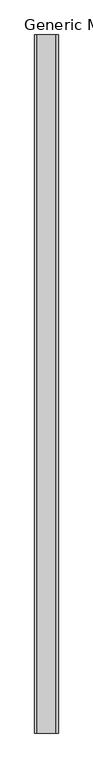
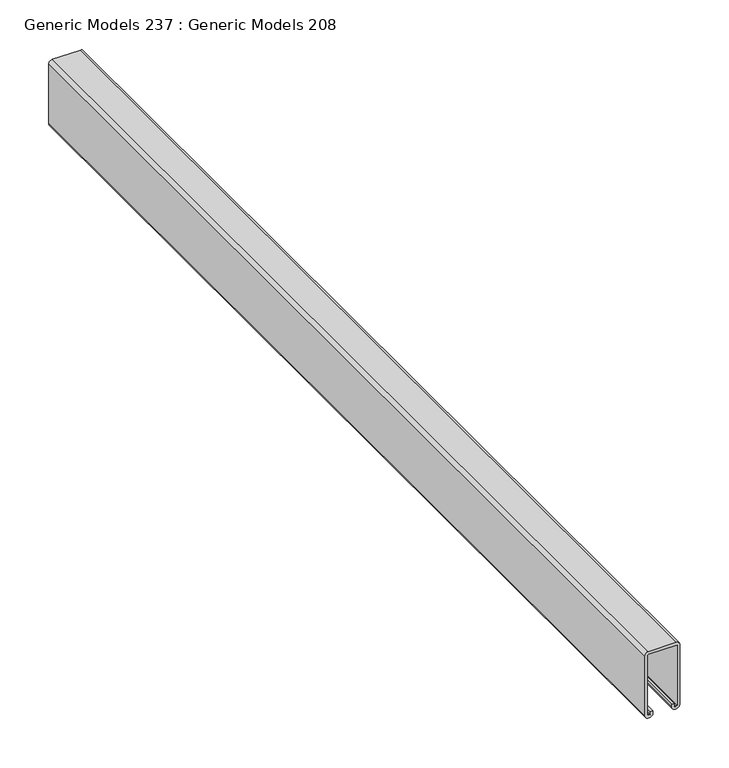
"""IFC4 building model written with IfcOpenShell, lengths in millimetres: proxy geometry, Generic Models 237 : Generic Models 208."""

import ifcopenshell
import ifcopenshell.guid

model = None  # the IFC model being written
_history = None  # IfcOwnerHistory: only IFC2X3 demands one
_inside = {}  # id of a spatial element -> (the spatial element, [elements in it])
_under = {}  # id of a project, library or spatial element -> (it, [spatial elements below it])
_declared = {}  # id of a project -> (the project, [libraries it declares])
_typed = {}  # id of a type object -> (the type object, [elements of that type])
_made_of = {}  # id of a material, layer set ... -> (it, [elements and type objects made of it])


def new_model(schema):
    """Start an empty IFC model of exactly this schema.

    Asked for "IFC4X3", IfcOpenShell would pick the latest addendum, in which some entities
    have other attributes; the version numbers below select the first issue.
    IFC2X3 requires an IfcOwnerHistory on every rooted entity: one is made here for all.
    """
    global model, _history
    if schema == "IFC4X3":
        model = ifcopenshell.file(schema_version=(4, 3, 0, 0))
    else:
        model = ifcopenshell.file(schema=schema)
    _inside.clear()
    _under.clear()
    _declared.clear()
    _typed.clear()
    _made_of.clear()
    _history = None
    if model.schema == "IFC2X3":
        org = make("IfcOrganization", Name="unknown")
        user = make(
            "IfcPersonAndOrganization",
            ThePerson=make("IfcPerson", FamilyName="unknown"),
            TheOrganization=org,
        )
        app = make(
            "IfcApplication",
            ApplicationDeveloper=org,
            Version="unknown",
            ApplicationFullName="unknown",
            ApplicationIdentifier="unknown",
        )
        _history = make(
            "IfcOwnerHistory",
            OwningUser=user,
            OwningApplication=app,
            ChangeAction="ADDED",
            CreationDate=0,
        )
    return model


def make(cls, **values):
    """One entity of the class cls with the attributes given. An attribute that is None is left unset."""
    return model.create_entity(
        cls, **{name: value for name, value in values.items() if value is not None}
    )


def rooted(cls, **values):
    """An entity with a GlobalId (a new one), such as an element, a storey or a relation."""
    return make(cls, GlobalId=ifcopenshell.guid.new(), OwnerHistory=_history, **values)


def si_unit(unit_type, name, prefix=None):
    """IfcSIUnit, for example si_unit("LENGTHUNIT", "METRE", prefix="MILLI")."""
    return make("IfcSIUnit", UnitType=unit_type, Prefix=prefix, Name=name)


def assignment(units):
    """IfcUnitAssignment: the units of a project."""
    return None if units is None else make("IfcUnitAssignment", Units=units)


def point(xyz):
    """IfcCartesianPoint."""
    return None if xyz is None else make("IfcCartesianPoint", Coordinates=xyz)


def direction(xyz):
    """IfcDirection."""
    return None if xyz is None else make("IfcDirection", DirectionRatios=xyz)


def frame(location, z_axis=None, x_axis=None):
    """IfcAxis2Placement3D, a coordinate frame: its origin and axes. An axis left out is left unset."""
    return make(
        "IfcAxis2Placement3D",
        Location=point(location),
        Axis=direction(z_axis),
        RefDirection=direction(x_axis),
    )


def frame_2d(location, x_axis=None):
    """IfcAxis2Placement2D, a coordinate frame in the plane: its origin and x axis."""
    return make(
        "IfcAxis2Placement2D", Location=point(location), RefDirection=direction(x_axis)
    )


def origin():
    """The frame at (0, 0, 0) with its axes left unset."""
    return frame((0.0, 0.0, 0.0))


def place(relative_to, where):
    """IfcLocalPlacement: puts the frame where relative to a parent placement (None: the world)."""
    return make(
        "IfcLocalPlacement", PlacementRelTo=relative_to, RelativePlacement=where
    )


def context(
    kind, dimensions, precision=None, world=None, true_north=None, identifier=None
):
    """IfcGeometricRepresentationContext, for example the 3D "Model" context."""
    return make(
        "IfcGeometricRepresentationContext",
        ContextIdentifier=identifier,
        ContextType=kind,
        CoordinateSpaceDimension=dimensions,
        Precision=precision,
        WorldCoordinateSystem=world,
        TrueNorth=true_north,
    )


def project(units=None, contexts=None):
    """IfcProject with its units and contexts."""
    return rooted(
        "IfcProject",
        Name="project",
        RepresentationContexts=contexts,
        UnitsInContext=assignment(units),
    )


def spatial(cls, under=None, at=None, **own):
    """A site, building, storey or space (cls), placed at a placement, below another one or the project."""
    s = rooted(cls, ObjectPlacement=at, **own)
    if under is not None:
        _under.setdefault(under.id(), (under, []))[1].append(s)
    return s


def polyline(points):
    """IfcPolyline through the points."""
    return make("IfcPolyline", Points=[point(p) for p in points])


def circle_curve(where, radius):
    """IfcCircle in the frame where."""
    return make("IfcCircle", Position=where, Radius=radius)


def trimmed(basis, trim1, trim2, sense, master):
    """IfcTrimmedCurve: the piece of a basis curve between two trims."""
    return make(
        "IfcTrimmedCurve",
        BasisCurve=basis,
        Trim1=trim1,
        Trim2=trim2,
        SenseAgreement=sense,
        MasterRepresentation=master,
    )


def segment(curve, same_sense, transition):
    """IfcCompositeCurveSegment."""
    return make(
        "IfcCompositeCurveSegment",
        Transition=transition,
        SameSense=same_sense,
        ParentCurve=curve,
    )


def composite_curve(segments, self_intersect=None):
    """IfcCompositeCurve: segments joined end to end."""
    return make("IfcCompositeCurve", Segments=segments, SelfIntersect=self_intersect)


def outline(outer, holes=None, kind="AREA"):
    """IfcArbitraryClosedProfileDef: a profile drawn as a closed curve; with holes, ...WithVoids."""
    if holes is None:
        return make("IfcArbitraryClosedProfileDef", ProfileType=kind, OuterCurve=outer)
    return make(
        "IfcArbitraryProfileDefWithVoids",
        ProfileType=kind,
        OuterCurve=outer,
        InnerCurves=holes,
    )


def extrude(swept, where, along, depth):
    """IfcExtrudedAreaSolid: the profile swept, set in the frame where, extruded along a direction by depth."""
    return make(
        "IfcExtrudedAreaSolid",
        SweptArea=swept,
        Position=where,
        ExtrudedDirection=direction(along),
        Depth=depth,
    )


def shape(context_of_items, identifier, shape_type, items):
    """IfcShapeRepresentation: the items that make up one representation, for example the "Body"."""
    return make(
        "IfcShapeRepresentation",
        ContextOfItems=context_of_items,
        RepresentationIdentifier=identifier,
        RepresentationType=shape_type,
        Items=items,
    )


def source(mapping_origin, context_of_items, identifier, shape_type, items):
    """IfcRepresentationMap: a shape defined once, which mapped items show again and again."""
    return make(
        "IfcRepresentationMap",
        MappingOrigin=mapping_origin,
        MappedRepresentation=shape(context_of_items, identifier, shape_type, items),
    )


def transform(
    local_origin,
    x_axis=None,
    y_axis=None,
    z_axis=None,
    scale=None,
    scale2=None,
    scale3=None,
    uniform=True,
):
    """IfcCartesianTransformationOperator3D, or its non-uniform kind. x_axis, y_axis, z_axis: its Axis1, 2, 3."""
    if uniform:
        return make(
            "IfcCartesianTransformationOperator3D",
            Axis1=direction(x_axis),
            Axis2=direction(y_axis),
            LocalOrigin=point(local_origin),
            Scale=scale,
            Axis3=direction(z_axis),
        )
    return make(
        "IfcCartesianTransformationOperator3DnonUniform",
        Axis1=direction(x_axis),
        Axis2=direction(y_axis),
        LocalOrigin=point(local_origin),
        Scale=scale,
        Axis3=direction(z_axis),
        Scale2=scale2,
        Scale3=scale3,
    )


def mapped(mapping_source, mapping_target):
    """IfcMappedItem: shows the shape of a source again, moved by a transform."""
    return make(
        "IfcMappedItem", MappingSource=mapping_source, MappingTarget=mapping_target
    )


def made_of(thing, what):
    """Note that an element or type object is made of a material, layer set ...; save() writes the relation."""
    if what is not None:
        _made_of.setdefault(what.id(), (what, []))[1].append(thing)
    return thing


def element(
    cls,
    number,
    at=None,
    inside=None,
    cuts=None,
    type_object=None,
    material=None,
    context=None,
    identifier="Body",
    shape_type=None,
    held_by="IfcProductDefinitionShape",
    body=None,
    shapes=None,
    **own,
):
    """One element of the class cls, such as IfcWall. Its Tag is "e" and its number.

    at: its placement. inside: the storey or other place that contains it. cuts: it is an
    opening in that element (IfcRelVoidsElement). A single representation is given by context,
    identifier, shape_type and body (its items); several are given by shapes. held_by: the class
    of the entity that holds the representations. save() writes the other relations.
    """
    e = rooted(cls, Tag="e%d" % number, ObjectPlacement=at, **own)
    if body is not None:
        shapes = [shape(context, identifier, shape_type, body)]
    if shapes is not None:
        e.Representation = make(held_by, Representations=shapes)
    if inside is not None:
        _inside.setdefault(inside.id(), (inside, []))[1].append(e)
    if cuts is not None:
        rooted(
            "IfcRelVoidsElement", RelatingBuildingElement=cuts, RelatedOpeningElement=e
        )
    if type_object is not None:
        _typed.setdefault(type_object.id(), (type_object, []))[1].append(e)
    return made_of(e, material)


def aggregate(whole, parts):
    """IfcRelAggregates: a whole, such as a stair, and the parts it consists of."""
    return rooted("IfcRelAggregates", RelatingObject=whole, RelatedObjects=parts)


def save(model, path):
    """Write the relations noted so far, then the file.

    IfcRelAggregates (storeys below a building ...), IfcRelContainedInSpatialStructure (elements
    in a storey), IfcRelDefinesByType, IfcRelAssociatesMaterial and IfcRelDeclares: one each for
    every whole, place, type object, material and project.
    """
    for whole, parts in _under.values():
        aggregate(whole, parts)
    for where, things in _inside.values():
        rooted(
            "IfcRelContainedInSpatialStructure",
            RelatedElements=things,
            RelatingStructure=where,
        )
    for kind, things in _typed.values():
        rooted("IfcRelDefinesByType", RelatedObjects=things, RelatingType=kind)
    for what, things in _made_of.values():
        rooted("IfcRelAssociatesMaterial", RelatedObjects=things, RelatingMaterial=what)
    for by, libraries in _declared.values():
        rooted("IfcRelDeclares", RelatingContext=by, RelatedDefinitions=libraries)
    model.write(path)


def generic_models_237_generic_models_208_3aec07af(model_context):
    return source(origin(), model_context, "Body", "SweptSolid", [
        extrude(outline(composite_curve([segment(polyline([(2050.797378, 53718.8649408), (2053.9878412, 53718.8649408), (2053.9878412, 53715.6899408), (2050.797378, 53715.6899408)]), True, "CONTINUOUS"), segment(trimmed(circle_curve(frame_2d((2050.797378, 53714.9116541)), 0.7782868), [point((2050.797378, 53715.6899408))], [point((2050.0190912, 53714.9116541))], True, "CARTESIAN"), True, "CONTINUOUS"), segment(polyline([(2050.0190912, 53714.9116541), (2050.0190912, 53713.3653996)]), True, "CONTINUOUS"), segment(trimmed(circle_curve(frame_2d((2050.86955, 53713.3653996)), 0.8504588), [point((2050.0190912, 53713.3653996))], [point((2050.86955, 53712.5149408))], True, "CARTESIAN"), True, "CONTINUOUS"), segment(polyline([(2050.86955, 53712.5149408), (2125.3702466, 53712.5149408)]), True, "CONTINUOUS"), segment(trimmed(circle_curve(frame_2d((2125.3702466, 53713.3637855)), 0.8488446), [point((2125.3702466, 53712.5149408))], [point((2126.2190912, 53713.3637855))], True, "CARTESIAN"), True, "CONTINUOUS"), segment(polyline([(2126.2190912, 53713.3637855), (2126.2190912, 53746.6306179)]), True, "CONTINUOUS"), segment(trimmed(circle_curve(frame_2d((2125.4097683, 53746.6306179)), 0.8093229), [point((2126.2190912, 53746.6306179))], [point((2125.4097683, 53747.4399408))], True, "CARTESIAN"), True, "CONTINUOUS"), segment(polyline([(2125.4097683, 53747.4399408), (2050.8560001, 53747.4399408)]), True, "CONTINUOUS"), segment(trimmed(circle_curve(frame_2d((2050.8560001, 53746.6030319)), 0.8369089), [point((2050.8560001, 53747.4399408))], [point((2050.0190912, 53746.6030319))], True, "CARTESIAN"), True, "CONTINUOUS"), segment(polyline([(2050.0190912, 53746.6030319), (2050.0190912, 53745.1342437)]), True, "CONTINUOUS"), segment(trimmed(circle_curve(frame_2d((2050.8883942, 53745.1342437)), 0.8693029), [point((2050.0190912, 53745.1342437))], [point((2050.8883942, 53744.2649408))], True, "CARTESIAN"), True, "CONTINUOUS"), segment(polyline([(2050.8883942, 53744.2649408), (2053.9878412, 53744.2649408), (2053.9878412, 53741.0899408), (2050.8883942, 53741.0899408)]), True, "CONTINUOUS"), segment(trimmed(circle_curve(frame_2d((2050.8883942, 53745.1342437)), 4.0443029), [point((2050.8883942, 53741.0899408))], [point((2046.8440912, 53745.1342437))], False, "CARTESIAN"), True, "CONTINUOUS"), segment(polyline([(2046.8440912, 53745.1342437), (2046.8440912, 53746.6030319)]), True, "CONTINUOUS"), segment(trimmed(circle_curve(frame_2d((2050.8560001, 53746.6030319)), 4.0119089), [point((2046.8440912, 53746.6030319))], [point((2050.8560001, 53750.6149408))], False, "CARTESIAN"), True, "CONTINUOUS"), segment(polyline([(2050.8560001, 53750.6149408), (2125.4097683, 53750.6149408)]), True, "CONTINUOUS"), segment(trimmed(circle_curve(frame_2d((2125.4097683, 53746.6306179)), 3.9843229), [point((2125.4097683, 53750.6149408))], [point((2129.3940912, 53746.6306179))], False, "CARTESIAN"), True, "CONTINUOUS"), segment(polyline([(2129.3940912, 53746.6306179), (2129.3940912, 53713.3637855)]), True, "CONTINUOUS"), segment(trimmed(circle_curve(frame_2d((2125.3702466, 53713.3637855)), 4.0238446), [point((2129.3940912, 53713.3637855))], [point((2125.3702466, 53709.3399408))], False, "CARTESIAN"), True, "CONTINUOUS"), segment(polyline([(2125.3702466, 53709.3399408), (2050.86955, 53709.3399408)]), True, "CONTINUOUS"), segment(trimmed(circle_curve(frame_2d((2050.86955, 53713.3653996)), 4.0254588), [point((2050.86955, 53709.3399408))], [point((2046.8440912, 53713.3653996))], False, "CARTESIAN"), True, "CONTINUOUS"), segment(polyline([(2046.8440912, 53713.3653996), (2046.8440912, 53714.9116541)]), True, "CONTINUOUS"), segment(trimmed(circle_curve(frame_2d((2050.797378, 53714.9116541)), 3.9532868), [point((2046.8440912, 53714.9116541))], [point((2050.797378, 53718.8649408))], False, "CARTESIAN"), True, "CONTINUOUS")], self_intersect=False)), frame((0.0, -228.7033818, 0.0), z_axis=(0.0, 1.0, 0.0), x_axis=(0.0, 0.0, 1.0)), (0.0, 0.0, 1.0), 1219.2),
    ])


if __name__ == "__main__":
    model = new_model("IFC4")
    model_context = context("Model", 3, world=origin())
    ifc_project = project(units=[si_unit("LENGTHUNIT", "METRE", prefix="MILLI")], contexts=[model_context])
    site = spatial("IfcSite", under=ifc_project)
    building = spatial("IfcBuilding", under=site)
    placement = place(None, origin())
    generic_models_237_generic_models_208_shape = generic_models_237_generic_models_208_3aec07af(model_context)
    element("IfcBuildingElementProxy", 1, Name="Generic Models 237 : Generic Models 208", ObjectType="Generic Models 237 : Generic Models 208", at=placement, inside=building, context=model_context, shape_type="MappedRepresentation", body=[
        mapped(generic_models_237_generic_models_208_shape, transform((0.0, 0.0, 0.0), x_axis=(1.0, 0.0, 0.0), y_axis=(0.0, 1.0, 0.0), z_axis=(0.0, 0.0, 1.0))),
    ])
    save(model, "model.ifc")

# Revit data of these elements
# Element 1 (IfcBuildingElementProxy, "Generic Models 237 : Generic Models 208")
#   Materials on its faces: "UNISTRUT P5000, 1-5/8\" x 3-1/4\", 12 GA METAL FRAMING CHANNEL STRUT"
# Materials
#   "UNISTRUT P5000, 1-5/8\" x 3-1/4\", 12 GA METAL FRAMING CHANNEL STRUT": class "Metal", colour RGB 244 244 244, transparency 0, Description = "Aluminum 6061", Cost = 0
